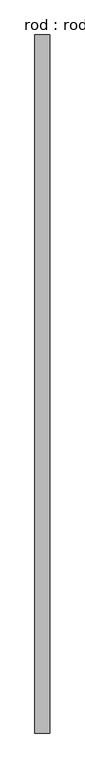
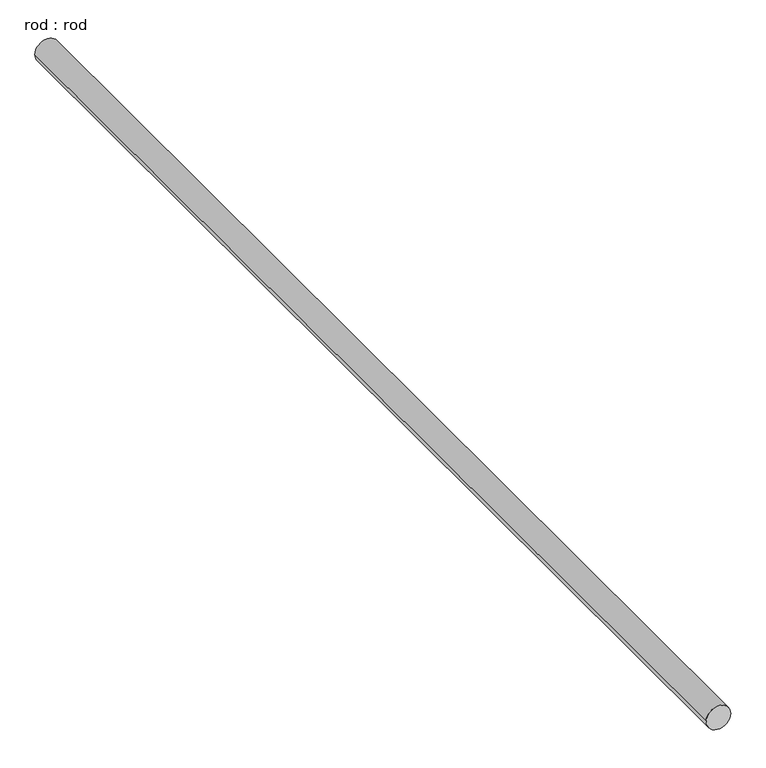
"""IFC4 building model written with IfcOpenShell, lengths in millimetres: proxy geometry, rod : rod."""

from ifc_helpers import new_model, si_unit, point, frame, frame_2d, origin, place, context, project, spatial, circle_curve, trimmed, segment, composite_curve, outline, extrude, source, transform, mapped, element, save


def rod_rod_61ade8de(model_context):
    return source(origin(), model_context, "Body", "SweptSolid", [
        extrude(outline(composite_curve([segment(trimmed(circle_curve(frame_2d((0.0108462, 0.0)), 200.0), [point((0.0108462, 200.0))], [point((0.0108462, -200.0))], False, "CARTESIAN"), True, "CONTINUOUS"), segment(trimmed(circle_curve(frame_2d((0.0108462, 0.0)), 200.0), [point((0.0108462, -200.0))], [point((0.0108462, 200.0))], False, "CARTESIAN"), True, "CONTINUOUS")], self_intersect=False)), frame((0.0, -5389.995479, 0.0), z_axis=(0.0, 1.0, 0.0), x_axis=(0.0, 0.0, 1.0)), (0.0, 0.0, 1.0), 18965.4481887),
    ])


if __name__ == "__main__":
    model = new_model("IFC4")
    model_context = context("Model", 3, world=origin())
    ifc_project = project(units=[si_unit("LENGTHUNIT", "METRE", prefix="MILLI")], contexts=[model_context])
    site = spatial("IfcSite", under=ifc_project)
    building = spatial("IfcBuilding", under=site)
    placement = place(None, origin())
    rod_rod_shape = rod_rod_61ade8de(model_context)
    element("IfcBuildingElementProxy", 1, Name="rod : rod", ObjectType="rod : rod", at=placement, inside=building, context=model_context, shape_type="MappedRepresentation", body=[
        mapped(rod_rod_shape, transform((0.0, 0.0, 0.0), x_axis=(1.0, 0.0, 0.0), y_axis=(0.0, 1.0, 0.0), z_axis=(0.0, 0.0, 1.0))),
    ])
    save(model, "model.ifc")

# Revit data of these elements
# Type "rod : rod"
#   Default Elevation = 0
